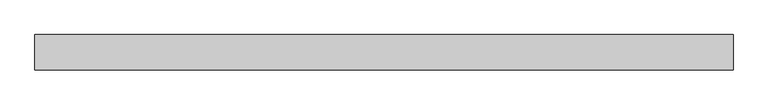
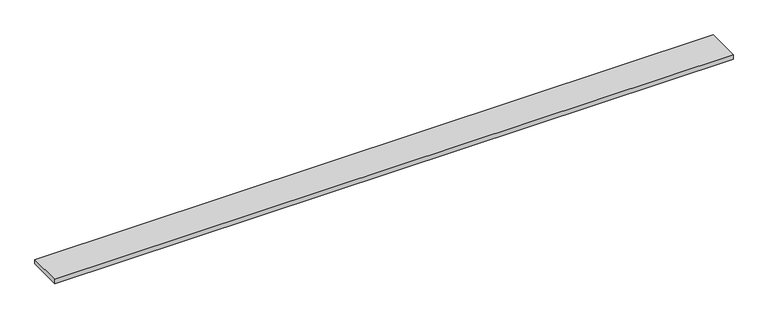
"""IFC4 building model written with IfcOpenShell, lengths in millimetres: proxy geometry, Generic Models 7:Generic Models 1:337419:Generic Models 1:337419 : Generic Models 7:Generic Models 1:337419:27 : Generic Models 7:Generic Models 1:337419:Generic Models 1:337419 : Generic Models 7:Generic Models 1:337419:301336."""

import ifcopenshell
import ifcopenshell.guid

model = None  # the IFC model being written
_history = None  # IfcOwnerHistory: only IFC2X3 demands one
_inside = {}  # id of a spatial element -> (the spatial element, [elements in it])
_under = {}  # id of a project, library or spatial element -> (it, [spatial elements below it])
_declared = {}  # id of a project -> (the project, [libraries it declares])
_typed = {}  # id of a type object -> (the type object, [elements of that type])
_made_of = {}  # id of a material, layer set ... -> (it, [elements and type objects made of it])


def new_model(schema):
    """Start an empty IFC model of exactly this schema.

    Asked for "IFC4X3", IfcOpenShell would pick the latest addendum, in which some entities
    have other attributes; the version numbers below select the first issue.
    IFC2X3 requires an IfcOwnerHistory on every rooted entity: one is made here for all.
    """
    global model, _history
    if schema == "IFC4X3":
        model = ifcopenshell.file(schema_version=(4, 3, 0, 0))
    else:
        model = ifcopenshell.file(schema=schema)
    _inside.clear()
    _under.clear()
    _declared.clear()
    _typed.clear()
    _made_of.clear()
    _history = None
    if model.schema == "IFC2X3":
        org = make("IfcOrganization", Name="unknown")
        user = make(
            "IfcPersonAndOrganization",
            ThePerson=make("IfcPerson", FamilyName="unknown"),
            TheOrganization=org,
        )
        app = make(
            "IfcApplication",
            ApplicationDeveloper=org,
            Version="unknown",
            ApplicationFullName="unknown",
            ApplicationIdentifier="unknown",
        )
        _history = make(
            "IfcOwnerHistory",
            OwningUser=user,
            OwningApplication=app,
            ChangeAction="ADDED",
            CreationDate=0,
        )
    return model


def make(cls, **values):
    """One entity of the class cls with the attributes given. An attribute that is None is left unset."""
    return model.create_entity(
        cls, **{name: value for name, value in values.items() if value is not None}
    )


def rooted(cls, **values):
    """An entity with a GlobalId (a new one), such as an element, a storey or a relation."""
    return make(cls, GlobalId=ifcopenshell.guid.new(), OwnerHistory=_history, **values)


def si_unit(unit_type, name, prefix=None):
    """IfcSIUnit, for example si_unit("LENGTHUNIT", "METRE", prefix="MILLI")."""
    return make("IfcSIUnit", UnitType=unit_type, Prefix=prefix, Name=name)


def assignment(units):
    """IfcUnitAssignment: the units of a project."""
    return None if units is None else make("IfcUnitAssignment", Units=units)


def point(xyz):
    """IfcCartesianPoint."""
    return None if xyz is None else make("IfcCartesianPoint", Coordinates=xyz)


def direction(xyz):
    """IfcDirection."""
    return None if xyz is None else make("IfcDirection", DirectionRatios=xyz)


def frame(location, z_axis=None, x_axis=None):
    """IfcAxis2Placement3D, a coordinate frame: its origin and axes. An axis left out is left unset."""
    return make(
        "IfcAxis2Placement3D",
        Location=point(location),
        Axis=direction(z_axis),
        RefDirection=direction(x_axis),
    )


def origin():
    """The frame at (0, 0, 0) with its axes left unset."""
    return frame((0.0, 0.0, 0.0))


def place(relative_to, where):
    """IfcLocalPlacement: puts the frame where relative to a parent placement (None: the world)."""
    return make(
        "IfcLocalPlacement", PlacementRelTo=relative_to, RelativePlacement=where
    )


def context(
    kind, dimensions, precision=None, world=None, true_north=None, identifier=None
):
    """IfcGeometricRepresentationContext, for example the 3D "Model" context."""
    return make(
        "IfcGeometricRepresentationContext",
        ContextIdentifier=identifier,
        ContextType=kind,
        CoordinateSpaceDimension=dimensions,
        Precision=precision,
        WorldCoordinateSystem=world,
        TrueNorth=true_north,
    )


def project(units=None, contexts=None):
    """IfcProject with its units and contexts."""
    return rooted(
        "IfcProject",
        Name="project",
        RepresentationContexts=contexts,
        UnitsInContext=assignment(units),
    )


def spatial(cls, under=None, at=None, **own):
    """A site, building, storey or space (cls), placed at a placement, below another one or the project."""
    s = rooted(cls, ObjectPlacement=at, **own)
    if under is not None:
        _under.setdefault(under.id(), (under, []))[1].append(s)
    return s


def polyline(points):
    """IfcPolyline through the points."""
    return make("IfcPolyline", Points=[point(p) for p in points])


def outline(outer, holes=None, kind="AREA"):
    """IfcArbitraryClosedProfileDef: a profile drawn as a closed curve; with holes, ...WithVoids."""
    if holes is None:
        return make("IfcArbitraryClosedProfileDef", ProfileType=kind, OuterCurve=outer)
    return make(
        "IfcArbitraryProfileDefWithVoids",
        ProfileType=kind,
        OuterCurve=outer,
        InnerCurves=holes,
    )


def extrude(swept, where, along, depth):
    """IfcExtrudedAreaSolid: the profile swept, set in the frame where, extruded along a direction by depth."""
    return make(
        "IfcExtrudedAreaSolid",
        SweptArea=swept,
        Position=where,
        ExtrudedDirection=direction(along),
        Depth=depth,
    )


def shape(context_of_items, identifier, shape_type, items):
    """IfcShapeRepresentation: the items that make up one representation, for example the "Body"."""
    return make(
        "IfcShapeRepresentation",
        ContextOfItems=context_of_items,
        RepresentationIdentifier=identifier,
        RepresentationType=shape_type,
        Items=items,
    )


def source(mapping_origin, context_of_items, identifier, shape_type, items):
    """IfcRepresentationMap: a shape defined once, which mapped items show again and again."""
    return make(
        "IfcRepresentationMap",
        MappingOrigin=mapping_origin,
        MappedRepresentation=shape(context_of_items, identifier, shape_type, items),
    )


def transform(
    local_origin,
    x_axis=None,
    y_axis=None,
    z_axis=None,
    scale=None,
    scale2=None,
    scale3=None,
    uniform=True,
):
    """IfcCartesianTransformationOperator3D, or its non-uniform kind. x_axis, y_axis, z_axis: its Axis1, 2, 3."""
    if uniform:
        return make(
            "IfcCartesianTransformationOperator3D",
            Axis1=direction(x_axis),
            Axis2=direction(y_axis),
            LocalOrigin=point(local_origin),
            Scale=scale,
            Axis3=direction(z_axis),
        )
    return make(
        "IfcCartesianTransformationOperator3DnonUniform",
        Axis1=direction(x_axis),
        Axis2=direction(y_axis),
        LocalOrigin=point(local_origin),
        Scale=scale,
        Axis3=direction(z_axis),
        Scale2=scale2,
        Scale3=scale3,
    )


def mapped(mapping_source, mapping_target):
    """IfcMappedItem: shows the shape of a source again, moved by a transform."""
    return make(
        "IfcMappedItem", MappingSource=mapping_source, MappingTarget=mapping_target
    )


def made_of(thing, what):
    """Note that an element or type object is made of a material, layer set ...; save() writes the relation."""
    if what is not None:
        _made_of.setdefault(what.id(), (what, []))[1].append(thing)
    return thing


def element(
    cls,
    number,
    at=None,
    inside=None,
    cuts=None,
    type_object=None,
    material=None,
    context=None,
    identifier="Body",
    shape_type=None,
    held_by="IfcProductDefinitionShape",
    body=None,
    shapes=None,
    **own,
):
    """One element of the class cls, such as IfcWall. Its Tag is "e" and its number.

    at: its placement. inside: the storey or other place that contains it. cuts: it is an
    opening in that element (IfcRelVoidsElement). A single representation is given by context,
    identifier, shape_type and body (its items); several are given by shapes. held_by: the class
    of the entity that holds the representations. save() writes the other relations.
    """
    e = rooted(cls, Tag="e%d" % number, ObjectPlacement=at, **own)
    if body is not None:
        shapes = [shape(context, identifier, shape_type, body)]
    if shapes is not None:
        e.Representation = make(held_by, Representations=shapes)
    if inside is not None:
        _inside.setdefault(inside.id(), (inside, []))[1].append(e)
    if cuts is not None:
        rooted(
            "IfcRelVoidsElement", RelatingBuildingElement=cuts, RelatedOpeningElement=e
        )
    if type_object is not None:
        _typed.setdefault(type_object.id(), (type_object, []))[1].append(e)
    return made_of(e, material)


def aggregate(whole, parts):
    """IfcRelAggregates: a whole, such as a stair, and the parts it consists of."""
    return rooted("IfcRelAggregates", RelatingObject=whole, RelatedObjects=parts)


def save(model, path):
    """Write the relations noted so far, then the file.

    IfcRelAggregates (storeys below a building ...), IfcRelContainedInSpatialStructure (elements
    in a storey), IfcRelDefinesByType, IfcRelAssociatesMaterial and IfcRelDeclares: one each for
    every whole, place, type object, material and project.
    """
    for whole, parts in _under.values():
        aggregate(whole, parts)
    for where, things in _inside.values():
        rooted(
            "IfcRelContainedInSpatialStructure",
            RelatedElements=things,
            RelatingStructure=where,
        )
    for kind, things in _typed.values():
        rooted("IfcRelDefinesByType", RelatedObjects=things, RelatingType=kind)
    for what, things in _made_of.values():
        rooted("IfcRelAssociatesMaterial", RelatedObjects=things, RelatingMaterial=what)
    for by, libraries in _declared.values():
        rooted("IfcRelDeclares", RelatingContext=by, RelatedDefinitions=libraries)
    model.write(path)


def generic_models_7370aaea(model_context):
    return source(origin(), model_context, "Body", "SweptSolid", [
        extrude(outline(polyline([(596182.8367242, -567935.4195091), (596182.8367242, -568183.8632591), (591306.0367242, -568183.8632591), (591306.0367242, -567935.4195091), (596182.8367242, -567935.4195091)])), frame((0.0, 0.0, 2489.1643609), z_axis=(0.0, 0.0, 1.0), x_axis=(1.0, 0.0, 0.0)), (0.0, 0.0, 1.0), 32.8770453),
    ])


if __name__ == "__main__":
    model = new_model("IFC4")
    model_context = context("Model", 3, world=origin())
    ifc_project = project(units=[si_unit("LENGTHUNIT", "METRE", prefix="MILLI")], contexts=[model_context])
    site = spatial("IfcSite", under=ifc_project)
    building = spatial("IfcBuilding", under=site)
    placement = place(None, origin())
    generic_models_shape = generic_models_7370aaea(model_context)
    element("IfcBuildingElementProxy", 1, Name="Generic Models 7:Generic Models 1:337419:Generic Models 1:337419 : Generic Models 7:Generic Models 1:337419:27 : Generic Models 7:Generic Models 1:337419:Generic Models 1:337419 : Generic Models 7:Generic Models 1:337419:301336", ObjectType="Generic Models 7:Generic Models 1:337419:Generic Models 1:337419 : Generic Models 7:Generic Models 1:337419:27 : Generic Models 7:Generic Models 1:337419:Generic Models 1:337419 : Generic Models 7:Generic Models 1:337419:301336", at=placement, inside=building, context=model_context, shape_type="MappedRepresentation", body=[
        mapped(generic_models_shape, transform((0.0, 0.0, 0.0), x_axis=(1.0, 0.0, 0.0), y_axis=(0.0, 1.0, 0.0), z_axis=(0.0, 0.0, 1.0))),
    ])
    save(model, "model.ifc")

# Revit data of these elements
# Type "Generic Models 7:Generic Models 1:337419:Generic Models 1:337419 : Generic Models 7:Generic Models 1:337419:27 : Generic Models 7:Generic Models 1:337419:Generic Models 1:337419 : Generic Models 7:Generic Models 1:337419:301336"
#   NameOverride = "Generic Models 7:Generic Models 1:337419:Generic Models 1:337419 : Generic Models 7:Generic Models 1:337419:301336"
#   ObjectTypeOverride = "Generic Models 1:337419 : Generic Models 7:Generic Models 1:337419"
#   Reference = "Generic Models 1"
#   Tag = "301336"
# Element 1 (IfcBuildingElementProxy, "Generic Models 7:Generic Models 1:337419:Generic Models 1:337419 : Generic Models 7:Generic Models 1:337419:27 : Generic Models 7:Generic Models 1:337419:Generic Models 1:337419 : Generic Models 7:Generic Models 1:337419:301336")
#   Materials on its faces: "ENGINEERED WOOD TRIM (LP SMARTSIDE)"
# Materials
#   "ENGINEERED WOOD TRIM (LP SMARTSIDE)": class "Wood", colour RGB 108 80 40, transparency 0, Description = "Pinus Echinata", Cost = 0
